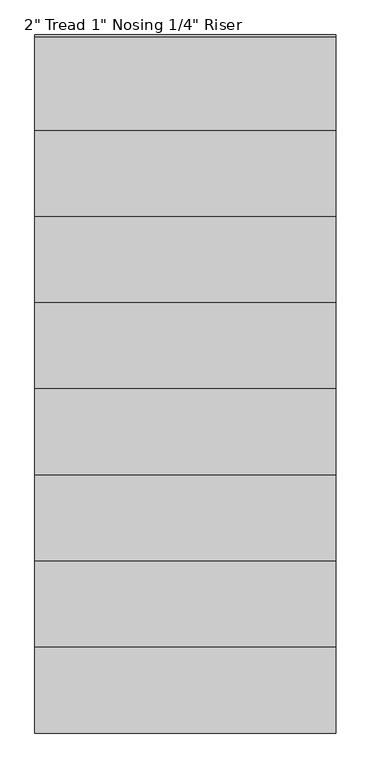
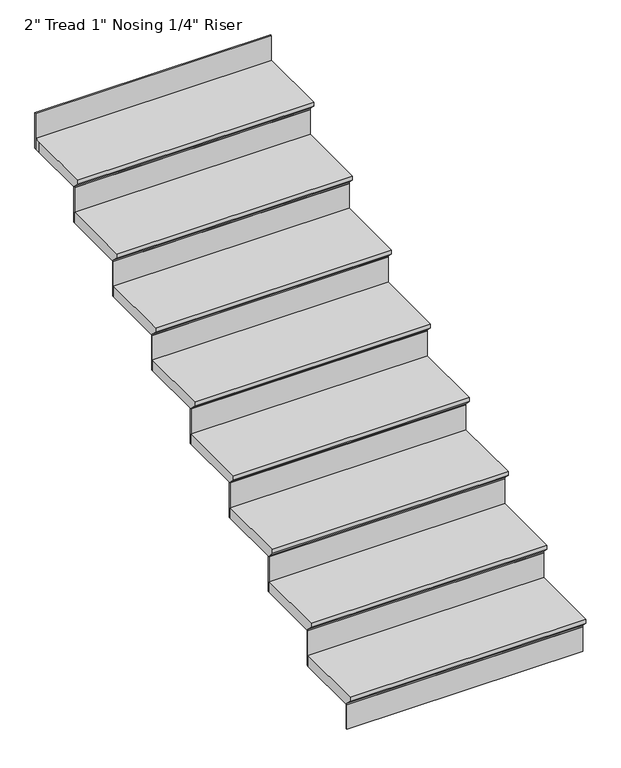
"""IFC4 building model written with IfcOpenShell, lengths in millimetres: stair flight geometry."""

from ifc_helpers import new_model, si_unit, origin, place, context, project, spatial, faceted_brep, source, transform, mapped, element, save


def stair_flight_ec5885e7(model_context):
    return source(origin(), model_context, "Body", "Brep", [
        faceted_brep([(37637.2404708, -15539.550078, 149.7852941), (37637.2404708, -15539.550078, 168.8352941), (36570.4404708, -15539.550078, 168.8352941), (36570.4404708, -15539.550078, 149.7852941), (37637.2404708, -15514.150078, 124.3852941), (36570.4404708, -15514.150078, 124.3852941), (37637.2404708, -15209.350078, 168.8352941), (36570.4404708, -15209.350078, 168.8352941), (36570.4404708, -15514.150078, 118.0352941), (36570.4404708, -15209.350078, 118.0352941), (37637.2404708, -15209.350078, 118.0352941), (37637.2404708, -15514.150078, 118.0352941)], [[[0, 1, 2, 3]], [[4, 0, 3, 5]], [[2, 1, 6, 7]], [[8, 9, 10, 11]], [[2, 7, 9, 8, 5, 3]], [[8, 11, 4, 5]], [[6, 1, 0, 4, 11, 10]], [[7, 6, 10, 9]]]),
        faceted_brep([(37637.2404708, -15514.150078, 118.0352941), (37637.2404708, -15514.150078, 0.0), (37637.2404708, -15507.800078, 0.0), (37637.2404708, -15507.800078, 118.0352941), (36570.4404708, -15514.150078, 118.0352941), (36570.4404708, -15507.800078, 118.0352941), (36570.4404708, -15507.800078, 0.0), (36570.4404708, -15514.150078, 0.0)], [[[0, 1, 2, 3]], [[4, 5, 6, 7]], [[1, 0, 4, 7]], [[2, 1, 7, 6]], [[3, 2, 6, 5]], [[0, 3, 5, 4]]]),
        faceted_brep([(37637.2404708, -15209.350078, 286.8705882), (37637.2404708, -15209.350078, 118.0352941), (37637.2404708, -15203.000078, 118.0352941), (37637.2404708, -15203.000078, 286.8705882), (36570.4404708, -15209.350078, 286.8705882), (36570.4404708, -15203.000078, 286.8705882), (36570.4404708, -15203.000078, 118.0352941), (36570.4404708, -15209.350078, 118.0352941)], [[[0, 1, 2, 3]], [[4, 5, 6, 7]], [[1, 0, 4, 7]], [[2, 1, 7, 6]], [[3, 2, 6, 5]], [[0, 3, 5, 4]]]),
        faceted_brep([(36570.4404708, -15234.750078, 337.6705882), (37637.2404708, -15234.750078, 337.6705882), (37637.2404708, -14904.550078, 337.6705882), (36570.4404708, -14904.550078, 337.6705882), (36570.4404708, -15209.350078, 286.8705882), (36570.4404708, -14904.550078, 286.8705882), (37637.2404708, -14904.550078, 286.8705882), (37637.2404708, -15209.350078, 286.8705882), (36570.4404708, -15209.350078, 293.2205882), (36570.4404708, -15234.750078, 318.6205882), (37637.2404708, -15209.350078, 293.2205882), (37637.2404708, -15234.750078, 318.6205882)], [[[0, 1, 2, 3]], [[4, 5, 6, 7]], [[0, 3, 5, 4, 8, 9]], [[4, 7, 10, 8]], [[2, 1, 11, 10, 7, 6]], [[3, 2, 6, 5]], [[11, 1, 0, 9]], [[10, 11, 9, 8]]]),
        faceted_brep([(37637.2404708, -14904.550078, 455.7058824), (37637.2404708, -14904.550078, 286.8705882), (37637.2404708, -14898.200078, 286.8705882), (37637.2404708, -14898.200078, 455.7058824), (36570.4404708, -14904.550078, 455.7058824), (36570.4404708, -14898.200078, 455.7058824), (36570.4404708, -14898.200078, 286.8705882), (36570.4404708, -14904.550078, 286.8705882)], [[[0, 1, 2, 3]], [[4, 5, 6, 7]], [[1, 0, 4, 7]], [[2, 1, 7, 6]], [[3, 2, 6, 5]], [[0, 3, 5, 4]]]),
        faceted_brep([(36570.4404708, -14929.950078, 506.5058824), (37637.2404708, -14929.950078, 506.5058824), (37637.2404708, -14599.750078, 506.5058824), (36570.4404708, -14599.750078, 506.5058824), (36570.4404708, -14904.550078, 455.7058824), (36570.4404708, -14599.750078, 455.7058824), (37637.2404708, -14599.750078, 455.7058824), (37637.2404708, -14904.550078, 455.7058824), (36570.4404708, -14904.550078, 462.0558824), (36570.4404708, -14929.950078, 487.4558824), (37637.2404708, -14904.550078, 462.0558824), (37637.2404708, -14929.950078, 487.4558824)], [[[0, 1, 2, 3]], [[4, 5, 6, 7]], [[0, 3, 5, 4, 8, 9]], [[4, 7, 10, 8]], [[2, 1, 11, 10, 7, 6]], [[3, 2, 6, 5]], [[11, 1, 0, 9]], [[10, 11, 9, 8]]]),
        faceted_brep([(37637.2404708, -14599.750078, 624.5411765), (37637.2404708, -14599.750078, 455.7058824), (37637.2404708, -14593.400078, 455.7058824), (37637.2404708, -14593.400078, 624.5411765), (36570.4404708, -14599.750078, 624.5411765), (36570.4404708, -14593.400078, 624.5411765), (36570.4404708, -14593.400078, 455.7058824), (36570.4404708, -14599.750078, 455.7058824)], [[[0, 1, 2, 3]], [[4, 5, 6, 7]], [[1, 0, 4, 7]], [[2, 1, 7, 6]], [[3, 2, 6, 5]], [[0, 3, 5, 4]]]),
        faceted_brep([(36570.4404708, -14625.150078, 675.3411765), (37637.2404708, -14625.150078, 675.3411765), (37637.2404708, -14294.950078, 675.3411765), (36570.4404708, -14294.950078, 675.3411765), (36570.4404708, -14599.750078, 624.5411765), (36570.4404708, -14294.950078, 624.5411765), (37637.2404708, -14294.950078, 624.5411765), (37637.2404708, -14599.750078, 624.5411765), (36570.4404708, -14599.750078, 630.8911765), (36570.4404708, -14625.150078, 656.2911765), (37637.2404708, -14599.750078, 630.8911765), (37637.2404708, -14625.150078, 656.2911765)], [[[0, 1, 2, 3]], [[4, 5, 6, 7]], [[0, 3, 5, 4, 8, 9]], [[4, 7, 10, 8]], [[2, 1, 11, 10, 7, 6]], [[3, 2, 6, 5]], [[11, 1, 0, 9]], [[10, 11, 9, 8]]]),
        faceted_brep([(37637.2404708, -14294.950078, 793.3764706), (37637.2404708, -14294.950078, 624.5411765), (37637.2404708, -14288.600078, 624.5411765), (37637.2404708, -14288.600078, 793.3764706), (36570.4404708, -14294.950078, 793.3764706), (36570.4404708, -14288.600078, 793.3764706), (36570.4404708, -14288.600078, 624.5411765), (36570.4404708, -14294.950078, 624.5411765)], [[[0, 1, 2, 3]], [[4, 5, 6, 7]], [[1, 0, 4, 7]], [[2, 1, 7, 6]], [[3, 2, 6, 5]], [[0, 3, 5, 4]]]),
        faceted_brep([(36570.4404708, -14320.350078, 844.1764706), (37637.2404708, -14320.350078, 844.1764706), (37637.2404708, -13990.150078, 844.1764706), (36570.4404708, -13990.150078, 844.1764706), (36570.4404708, -14294.950078, 793.3764706), (36570.4404708, -13990.150078, 793.3764706), (37637.2404708, -13990.150078, 793.3764706), (37637.2404708, -14294.950078, 793.3764706), (36570.4404708, -14294.950078, 799.7264706), (36570.4404708, -14320.350078, 825.1264706), (37637.2404708, -14294.950078, 799.7264706), (37637.2404708, -14320.350078, 825.1264706)], [[[0, 1, 2, 3]], [[4, 5, 6, 7]], [[0, 3, 5, 4, 8, 9]], [[4, 7, 10, 8]], [[2, 1, 11, 10, 7, 6]], [[3, 2, 6, 5]], [[11, 1, 0, 9]], [[10, 11, 9, 8]]]),
        faceted_brep([(37637.2404708, -13990.150078, 962.2117647), (37637.2404708, -13990.150078, 793.3764706), (37637.2404708, -13983.800078, 793.3764706), (37637.2404708, -13983.800078, 962.2117647), (36570.4404708, -13990.150078, 962.2117647), (36570.4404708, -13983.800078, 962.2117647), (36570.4404708, -13983.800078, 793.3764706), (36570.4404708, -13990.150078, 793.3764706)], [[[0, 1, 2, 3]], [[4, 5, 6, 7]], [[1, 0, 4, 7]], [[2, 1, 7, 6]], [[3, 2, 6, 5]], [[0, 3, 5, 4]]]),
        faceted_brep([(36570.4404708, -14015.550078, 1013.0117647), (37637.2404708, -14015.550078, 1013.0117647), (37637.2404708, -13685.350078, 1013.0117647), (36570.4404708, -13685.350078, 1013.0117647), (36570.4404708, -13990.150078, 962.2117647), (36570.4404708, -13685.350078, 962.2117647), (37637.2404708, -13685.350078, 962.2117647), (37637.2404708, -13990.150078, 962.2117647), (36570.4404708, -13990.150078, 968.5617647), (36570.4404708, -14015.550078, 993.9617647), (37637.2404708, -13990.150078, 968.5617647), (37637.2404708, -14015.550078, 993.9617647)], [[[0, 1, 2, 3]], [[4, 5, 6, 7]], [[0, 3, 5, 4, 8, 9]], [[4, 7, 10, 8]], [[2, 1, 11, 10, 7, 6]], [[3, 2, 6, 5]], [[11, 1, 0, 9]], [[10, 11, 9, 8]]]),
        faceted_brep([(37637.2404708, -13685.350078, 1131.0470588), (37637.2404708, -13685.350078, 962.2117647), (37637.2404708, -13679.000078, 962.2117647), (37637.2404708, -13679.000078, 1131.0470588), (36570.4404708, -13685.350078, 1131.0470588), (36570.4404708, -13679.000078, 1131.0470588), (36570.4404708, -13679.000078, 962.2117647), (36570.4404708, -13685.350078, 962.2117647)], [[[0, 1, 2, 3]], [[4, 5, 6, 7]], [[1, 0, 4, 7]], [[2, 1, 7, 6]], [[3, 2, 6, 5]], [[0, 3, 5, 4]]]),
        faceted_brep([(36570.4404708, -13710.750078, 1181.8470588), (37637.2404708, -13710.750078, 1181.8470588), (37637.2404708, -13380.550078, 1181.8470588), (36570.4404708, -13380.550078, 1181.8470588), (36570.4404708, -13685.350078, 1131.0470588), (36570.4404708, -13380.550078, 1131.0470588), (37637.2404708, -13380.550078, 1131.0470588), (37637.2404708, -13685.350078, 1131.0470588), (36570.4404708, -13685.350078, 1137.3970588), (36570.4404708, -13710.750078, 1162.7970588), (37637.2404708, -13685.350078, 1137.3970588), (37637.2404708, -13710.750078, 1162.7970588)], [[[0, 1, 2, 3]], [[4, 5, 6, 7]], [[0, 3, 5, 4, 8, 9]], [[4, 7, 10, 8]], [[2, 1, 11, 10, 7, 6]], [[3, 2, 6, 5]], [[11, 1, 0, 9]], [[10, 11, 9, 8]]]),
        faceted_brep([(37637.2404708, -13075.750078, 1468.7176471), (37637.2404708, -13075.750078, 1299.8823529), (37637.2404708, -13069.400078, 1299.8823529), (37637.2404708, -13069.400078, 1468.7176471), (36570.4404708, -13075.750078, 1468.7176471), (36570.4404708, -13069.400078, 1468.7176471), (36570.4404708, -13069.400078, 1299.8823529), (36570.4404708, -13075.750078, 1299.8823529)], [[[0, 1, 2, 3]], [[4, 5, 6, 7]], [[1, 0, 4, 7]], [[2, 1, 7, 6]], [[3, 2, 6, 5]], [[0, 3, 5, 4]]]),
        faceted_brep([(37637.2404708, -13380.550078, 1299.8823529), (37637.2404708, -13380.550078, 1131.0470588), (37637.2404708, -13374.200078, 1131.0470588), (37637.2404708, -13374.200078, 1299.8823529), (36570.4404708, -13380.550078, 1299.8823529), (36570.4404708, -13374.200078, 1299.8823529), (36570.4404708, -13374.200078, 1131.0470588), (36570.4404708, -13380.550078, 1131.0470588)], [[[0, 1, 2, 3]], [[4, 5, 6, 7]], [[1, 0, 4, 7]], [[2, 1, 7, 6]], [[3, 2, 6, 5]], [[0, 3, 5, 4]]]),
        faceted_brep([(36570.4404708, -13075.750078, 1350.6823529), (36570.4404708, -13101.150078, 1350.6823529), (36570.4404708, -13405.950078, 1350.6823529), (37637.2404708, -13405.950078, 1350.6823529), (37637.2404708, -13075.750078, 1350.6823529), (36570.4404708, -13101.150078, 1299.8823529), (36570.4404708, -13075.750078, 1299.8823529), (37637.2404708, -13075.750078, 1299.8823529), (37637.2404708, -13380.550078, 1299.8823529), (36570.4404708, -13380.550078, 1299.8823529), (36570.4404708, -13380.550078, 1306.2323529), (36570.4404708, -13405.950078, 1331.6323529), (37637.2404708, -13380.550078, 1306.2323529), (37637.2404708, -13405.950078, 1331.6323529)], [[[0, 1, 2, 3, 4]], [[5, 6, 7, 8, 9]], [[1, 0, 6, 5]], [[2, 1, 5, 9, 10, 11]], [[9, 8, 12, 10]], [[4, 3, 13, 12, 8, 7]], [[0, 4, 7, 6]], [[13, 3, 2, 11]], [[12, 13, 11, 10]]]),
    ])


if __name__ == "__main__":
    model = new_model("IFC4")
    model_context = context("Model", 3, world=origin())
    ifc_project = project(units=[si_unit("LENGTHUNIT", "METRE", prefix="MILLI")], contexts=[model_context])
    site = spatial("IfcSite", under=ifc_project)
    building = spatial("IfcBuilding", under=site)
    placement = place(None, origin())
    stair_flight_shape = stair_flight_ec5885e7(model_context)
    element("IfcStairFlight", 1, ObjectType="2\" Tread 1\" Nosing 1/4\" Riser", at=placement, inside=building, context=model_context, shape_type="MappedRepresentation", body=[
        mapped(stair_flight_shape, transform((0.0, 0.0, 0.0), x_axis=(1.0, 0.0, 0.0), y_axis=(0.0, 1.0, 0.0), z_axis=(0.0, 0.0, 1.0))),
    ])
    save(model, "model.ifc")

# Revit data of these elements
# Element 1 (IfcStairFlight, "2\" Tread 1\" Nosing 1/4\" Riser")
#   Materials on its faces: "Oak Flooring", "Wood Planks"
# Materials
#   "Oak Flooring": class "Wood", colour RGB 216 169 114, transparency 0, Description = "Quercus Rubra", Cost = 0
#   "Wood Planks": class "Wood", colour RGB 129 72 39, transparency 0, Description = "Physical material.", Cost = 0
